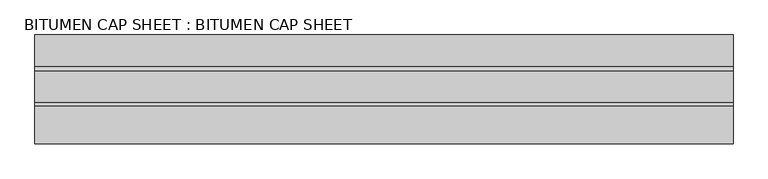
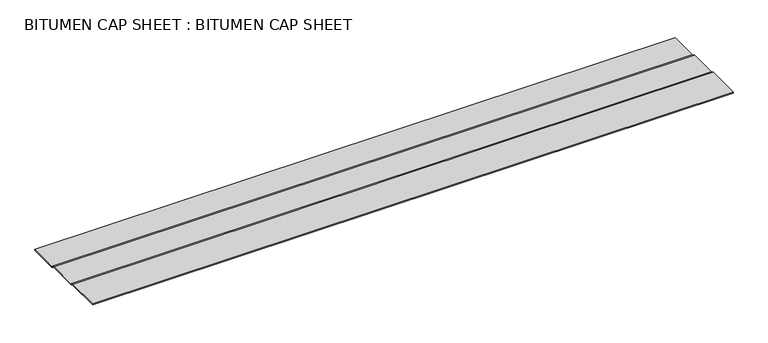
"""IFC4 building model written with IfcOpenShell, lengths in millimetres: proxy geometry, BITUMEN CAP SHEET : BITUMEN CAP SHEET."""

from ifc_helpers import new_model, si_unit, frame, origin, place, context, project, spatial, polyline, outline, extrude, source, transform, mapped, element, save


def bitumen_cap_sheet_bitumen_cap_sheet_a55ad838(model_context):
    return source(origin(), model_context, "Body", "SweptSolid", [
        extrude(outline(polyline([(-5237.2758356, 40238.7580714), (-5329.4404972, 40238.7580714), (-5341.9053158, 40244.0440809), (-5432.619472, 40244.0440809), (-5442.3358585, 40248.3766459), (-5549.5470696, 40248.3766459), (-5549.5470696, 40251.5518755), (-5441.660573, 40251.5518755), (-5431.9436715, 40247.2190809), (-5341.2599159, 40247.2190809), (-5328.7950972, 40241.9330714), (-5237.2758356, 40241.9330714), (-5237.2758356, 40238.7580714)])), frame((12382.7678845, 0.0, 0.0), z_axis=(1.0, 0.0, 0.0), x_axis=(0.0, 1.0, 0.0)), (0.0, 0.0, 1.0), 2000.25),
    ])


if __name__ == "__main__":
    model = new_model("IFC4")
    model_context = context("Model", 3, world=origin())
    ifc_project = project(units=[si_unit("LENGTHUNIT", "METRE", prefix="MILLI")], contexts=[model_context])
    site = spatial("IfcSite", under=ifc_project)
    building = spatial("IfcBuilding", under=site)
    placement = place(None, origin())
    bitumen_cap_sheet_bitumen_cap_sheet_shape = bitumen_cap_sheet_bitumen_cap_sheet_a55ad838(model_context)
    element("IfcBuildingElementProxy", 1, Name="BITUMEN CAP SHEET : BITUMEN CAP SHEET", ObjectType="BITUMEN CAP SHEET : BITUMEN CAP SHEET", at=placement, inside=building, context=model_context, shape_type="MappedRepresentation", body=[
        mapped(bitumen_cap_sheet_bitumen_cap_sheet_shape, transform((0.0, 0.0, 0.0), x_axis=(1.0, 0.0, 0.0), y_axis=(0.0, 1.0, 0.0), z_axis=(0.0, 0.0, 1.0))),
    ])
    save(model, "model.ifc")

# Revit data of these elements
# Type "BITUMEN CAP SHEET : BITUMEN CAP SHEET"
#   NameOverride = "BITUMEN CAP SHEET"
# Element 1 (IfcBuildingElementProxy, "BITUMEN CAP SHEET : BITUMEN CAP SHEET")
#   Materials on its faces: "MODIFIED BITUMEN GRANULE SURFACED CAP SHEET"
# Materials
#   "MODIFIED BITUMEN GRANULE SURFACED CAP SHEET": class "Unassigned", colour RGB 85 85 127, transparency 0
